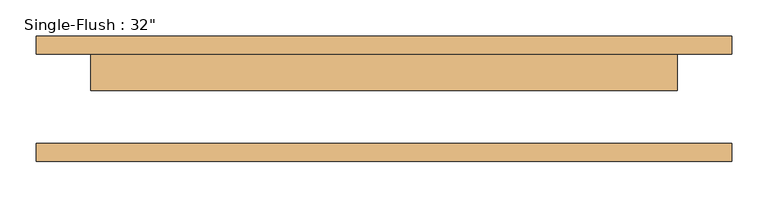
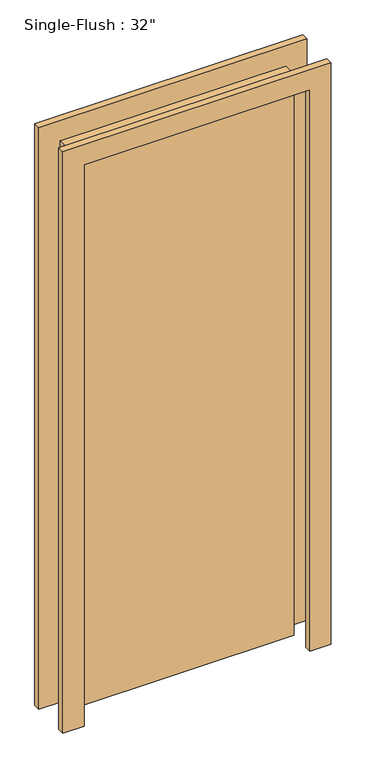
"""IFC4 building model written with IfcOpenShell, lengths in millimetres: door geometry."""

from ifc_helpers import new_model, si_unit, frame, origin, origin_with_axes, place, context, project, spatial, polyline, outline, extrude, source, transform, mapped, element, save


def door_8a652669(model_context):
    return source(origin(), model_context, "Body", "SweptSolid", [
        extrude(outline(polyline([(2209.8, -482.6), (0.0, -482.6), (0.0, -406.4), (2133.6, -406.4), (2133.6, 406.4), (0.0, 406.4), (0.0, 482.6), (2209.8, 482.6), (2209.8, -482.6)])), frame((0.0, 61.9125, 0.0), z_axis=(0.0, 1.0, 0.0), x_axis=(0.0, 0.0, 1.0)), (0.0, 0.0, 1.0), 25.4),
        extrude(outline(polyline([(2209.8, 482.6), (2209.8, -482.6), (0.0, -482.6), (0.0, -406.4), (2133.6, -406.4), (2133.6, 406.4), (0.0, 406.4), (0.0, 482.6), (2209.8, 482.6)])), frame((0.0, -87.3125, 0.0), z_axis=(0.0, 1.0, 0.0), x_axis=(0.0, 0.0, 1.0)), (0.0, 0.0, 1.0), 25.4),
        extrude(outline(polyline([(406.4, 11.1125), (-406.4, 11.1125), (-406.4, 61.9125), (406.4, 61.9125), (406.4, 11.1125)])), origin_with_axes(), (0.0, 0.0, 1.0), 2133.6),
    ])


if __name__ == "__main__":
    model = new_model("IFC4")
    model_context = context("Model", 3, world=origin())
    ifc_project = project(units=[si_unit("LENGTHUNIT", "METRE", prefix="MILLI")], contexts=[model_context])
    site = spatial("IfcSite", under=ifc_project)
    building = spatial("IfcBuilding", under=site)
    placement = place(None, origin())
    door_shape = door_8a652669(model_context)
    element("IfcDoor", 1, ObjectType="Single-Flush : 32\"", at=placement, inside=building, context=model_context, shape_type="MappedRepresentation", body=[
        mapped(door_shape, transform((0.0, 0.0, 0.0), x_axis=(1.0, 0.0, 0.0), y_axis=(0.0, 1.0, 0.0), z_axis=(0.0, 0.0, 1.0))),
    ])
    save(model, "model.ifc")

# Revit data of these elements
# Type "Single-Flush : 32\""
#   Type Mark = "57"
#   Construction Type Id = "MDOOR"
#   Assembly Code = "C1020"
#   Analytic Construction = "Metal"
#   Thickness = 0' - 2"
#   Heat Transfer Coefficient (U) = 3.7021 W/(m²·K)
#   Height = 7' - 0"
#   Trim Projection Ext = 0' - 1"
#   Trim Projection Int = 0' - 1"
#   Trim Width = 0' - 3"
#   Width = 2' - 8"
#   Door Material = Door - Panel
#   Frame Material = Door - Frame
#   Visual Light Transmittance = 0
#   Solar Heat Gain Coefficient = 0
#   Function = (empty or 0)
#   Wall Closure = (empty or 0)
# Element 1 (IfcDoor, "Single-Flush : 32\"")
#   Materials on its faces: "Door - Frame", "Door - Panel"
# Materials
#   "Door - Panel": class "Wood", colour RGB 210 159 95, transparency 0
#   "Door - Frame": class "Miscellaneous", colour RGB 118 70 51, transparency 0
